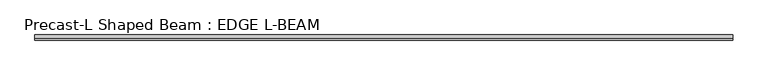
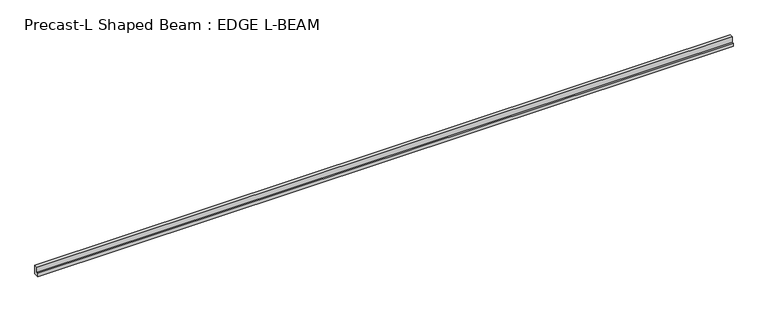
"""IFC4 building model written with IfcOpenShell, lengths in millimetres: beam geometry, Precast-L Shaped Beam : EDGE L-BEAM."""

from ifc_helpers import new_model, si_unit, frame, origin, place, context, project, spatial, polyline, outline, extrude, source, transform, mapped, element, save


def precast_l_shaped_beam_edge_l_beam_af089dbf(model_context):
    return source(origin(), model_context, "Body", "SweptSolid", [
        extrude(outline(polyline([(228.6, -406.4), (-228.6, -406.4), (-228.6, -101.6), (-76.2, -101.6), (-76.2, 406.4), (228.6, 406.4), (228.6, -406.4)])), frame((-31242.0, 0.0, 0.0), z_axis=(1.0, 0.0, 0.0), x_axis=(0.0, 1.0, 0.0)), (0.0, 0.0, 1.0), 62484.0),
    ])


if __name__ == "__main__":
    model = new_model("IFC4")
    model_context = context("Model", 3, world=origin())
    ifc_project = project(units=[si_unit("LENGTHUNIT", "METRE", prefix="MILLI")], contexts=[model_context])
    site = spatial("IfcSite", under=ifc_project)
    building = spatial("IfcBuilding", under=site)
    placement = place(None, origin())
    precast_l_shaped_beam_edge_l_beam_shape = precast_l_shaped_beam_edge_l_beam_af089dbf(model_context)
    element("IfcBeam", 1, ObjectType="Precast-L Shaped Beam : EDGE L-BEAM", at=placement, inside=building, context=model_context, shape_type="MappedRepresentation", body=[
        mapped(precast_l_shaped_beam_edge_l_beam_shape, transform((0.0, 0.0, 0.0), x_axis=(1.0, 0.0, 0.0), y_axis=(0.0, 1.0, 0.0), z_axis=(0.0, 0.0, 1.0))),
    ])
    save(model, "model.ifc")

# Revit data of these elements
# Type "Precast-L Shaped Beam : EDGE L-BEAM"
#   Assembly Code = "B10"
#   Seat = 0' - 6"
#   Length [instance default] = 5' - 0"
#   b = 1' - 6"
#   h = 2' - 8"
#   h1 = 1' - 8"
#   Structural Material [instance default] = Concrete, Precast
# Element 1 (IfcBeam, "Precast-L Shaped Beam : EDGE L-BEAM")
#   Length = 205' - 0"
#   Structural Material = Concrete - Precast Concrete - Normal Weight Concrete - 5 ksi
#   Materials on its faces: "Concrete - Precast Concrete - Normal Weight Concrete - 5 ksi"
# Materials
#   "Concrete, Precast": class "Concrete", colour RGB 198 187 187, transparency 0, Description = "Precast concrete", Cost = 0
#   "Concrete - Precast Concrete - Normal Weight Concrete - 5 ksi": class "Concrete", colour RGB 198 187 187, transparency 0, Cost = 0
